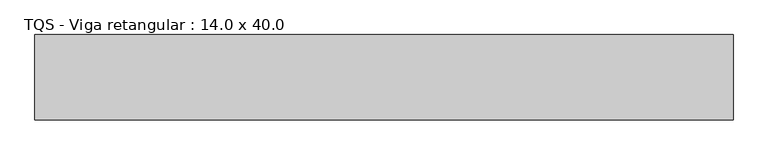
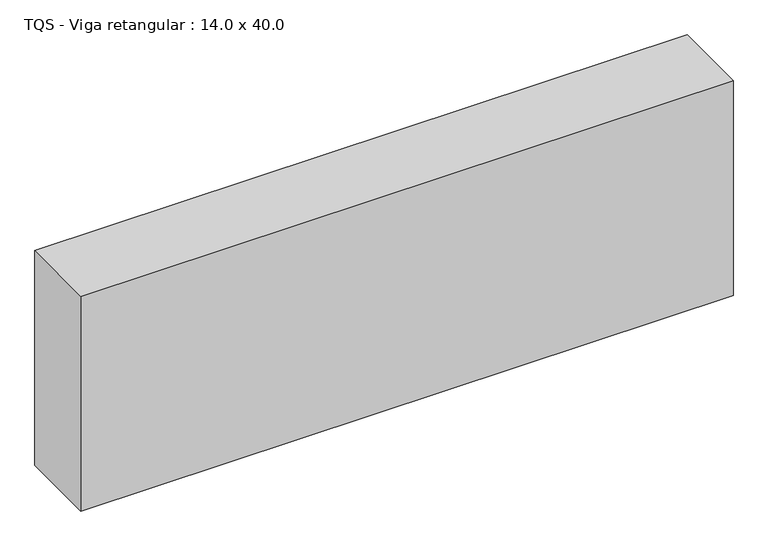
"""IFC4 building model written with IfcOpenShell, lengths in millimetres: beam geometry, TQS - Viga retangular : 14.0 x 40.0."""

from ifc_helpers import new_model, si_unit, frame, origin, place, context, project, spatial, polyline, outline, extrude, source, transform, mapped, element, save


def tqs_viga_retangular_14_0_x_40_0_8fae01fb(model_context):
    return source(origin(), model_context, "Body", "SweptSolid", [
        extrude(outline(polyline([(573.9, 70.0), (573.9, -70.0), (-573.9, -70.0), (-573.9, 70.0), (573.9, 70.0)])), frame((0.0, 0.0, -200.0), z_axis=(0.0, 0.0, 1.0), x_axis=(1.0, 0.0, 0.0)), (0.0, 0.0, 1.0), 400.0),
    ])


if __name__ == "__main__":
    model = new_model("IFC4")
    model_context = context("Model", 3, world=origin())
    ifc_project = project(units=[si_unit("LENGTHUNIT", "METRE", prefix="MILLI")], contexts=[model_context])
    site = spatial("IfcSite", under=ifc_project)
    building = spatial("IfcBuilding", under=site)
    placement = place(None, origin())
    tqs_viga_retangular_14_0_x_40_0_shape = tqs_viga_retangular_14_0_x_40_0_8fae01fb(model_context)
    element("IfcBeam", 1, ObjectType="TQS - Viga retangular : 14.0 x 40.0", at=placement, inside=building, context=model_context, shape_type="MappedRepresentation", body=[
        mapped(tqs_viga_retangular_14_0_x_40_0_shape, transform((0.0, 0.0, 0.0), x_axis=(1.0, 0.0, 0.0), y_axis=(0.0, 1.0, 0.0), z_axis=(0.0, 0.0, 1.0))),
    ])
    save(model, "model.ifc")

# Revit data of these elements
# Type "TQS - Viga retangular : 14.0 x 40.0"
#   Length [instance default] = 1.524 m
#   b = 0.14 m
#   h = 0.40 m
#   Structural Material [instance default] = none
#   Assembly Code = ""
